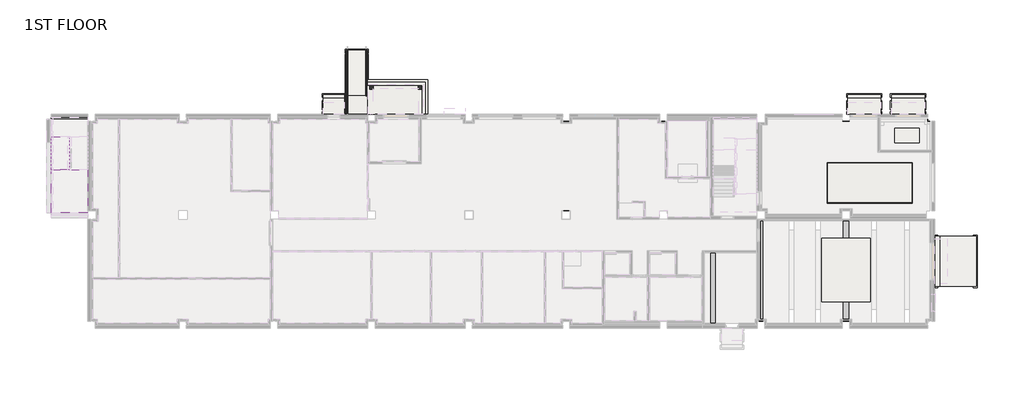
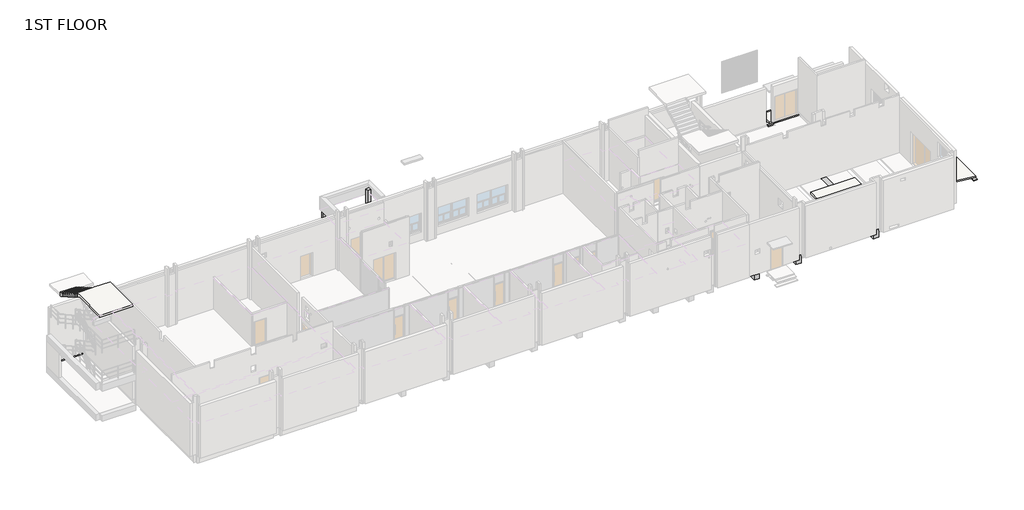
# One storey, part 10 of 15: 37 slabs, 9 beams, 2 columns, 1 stair flight.
# Revit data of these elements (continued)
# Elements 26, 31, 39, 43 (IfcSlab, "H_SF_AR_S18_Lean_T50") (continued)
#   Height Offset From Level = -350 mm
#   built-in parameter 1001954 = 1
#   Phase Created = New Construction
#   Materials on its faces: "Concrete_f'c=14MPa(Cylender)"
# Elements 27, 32, 41 (IfcSlab, "H_SF_AR_S18_Lean_T50")
#   Comments = ""
#   Height Offset From Level = -200 mm
#   built-in parameter 1001954 = 1
#   Phase Created = New Construction
#   Materials on its faces: "Concrete_f'c=14MPa(Cylender)"
# Element 33 (IfcSlab, "H_SF_AR_B08_Stoop_T150")
#   Comments = ""
#   Height Offset From Level = -20 mm
#   built-in parameter 1001954 = 1
#   Phase Created = New Construction
#   Materials on its faces: "Concrete_f'c=28MPa(Cylender)"
# Element 34 (IfcSlab, "H_SF_AR_B08_Stoop_T125")
#   Comments = ""
#   Height Offset From Level = -160 mm
#   built-in parameter 1001954 = 1
#   Phase Created = New Construction
#   Materials on its faces: "Concrete_f'c=28MPa(Cylender)"
# Element 35 (IfcSlab, "H_SF_AR_S18_Lean_T50")
#   Comments = ""
#   Height Offset From Level = -470 mm
#   built-in parameter 1001954 = 1
#   Phase Created = New Construction
#   Materials on its faces: "Concrete_f'c=14MPa(Cylender)"
# Element 36 (IfcSlab, "H_SF_AR_S18_Lean_T50")
#   Comments = ""
#   Height Offset From Level = -320 mm
#   built-in parameter 1001954 = 1
#   Phase Created = New Construction
#   Materials on its faces: "Concrete_f'c=14MPa(Cylender)"
# Element 37 (IfcSlab, "H_SF_AR_S18_Lean_T50")
#   Comments = ""
#   Height Offset From Level = -170 mm
#   built-in parameter 1001954 = 1
#   Phase Created = New Construction
#   Materials on its faces: "Concrete_f'c=14MPa(Cylender)"
# Element 40 (IfcSlab, "H_SF_AR_S18_Lean_T50")
#   Comments = ""
#   Height Offset From Level = -620.333 mm
#   built-in parameter 1001954 = 1
#   Phase Created = New Construction
#   Materials on its faces: "Concrete_f'c=14MPa(Cylender)"
# Element 42 (IfcSlab, "H_SF_AR_S18_Lean_T50")
#   Comments = ""
#   built-in parameter 1001955 = 3.14159 (stored number, unit not read)
#   Height Offset From Level = -350 mm
#   built-in parameter 1001954 = 1
#   Phase Created = New Construction
#   Materials on its faces: "Concrete_f'c=14MPa(Cylender)"
# Elements 44, 45 (IfcSlab, "H_SF_AR_S18_Lean_T50")
#   Comments = ""
#   built-in parameter 1001955 = -1.5708 (stored number, unit not read)
#   Height Offset From Level = -150 mm
#   built-in parameter 1001954 = 1
#   Phase Created = New Construction
#   Materials on its faces: "Concrete_f'c=14MPa(Cylender)"
# Element 46 (IfcSlab, "H_SF_AR_S18_Lean_T50")
#   Comments = ""
#   Height Offset From Level = -450 mm
#   built-in parameter 1001954 = 1
#   Phase Created = New Construction
#   Materials on its faces: "Concrete_f'c=14MPa(Cylender)"
# Element 48 (IfcSlab, "H_SF_AR_S18_Lean_T50")
#   Comments = ""
#   Height Offset From Level = -600 mm
#   built-in parameter 1001954 = 1
#   Phase Created = New Construction
#   Materials on its faces: "Concrete_f'c=14MPa(Cylender)"
# Element 49 (IfcStairFlight, "Concrete")
#   Phase Created = New Construction
#   Materials on its faces: "Concrete_f'c=28MPa(Cylender)"
# Materials
#   "Concrete_f'c=28MPa(Cylender)": class "Concrete", colour RGB 176 176 176, transparency 0, Description = "Reinf. Conc.", Cost = 0, Image = Concrete.Cast-In-Place.Flat.Polished.Grey.jpg
#   "Concrete_f'c=14MPa(Cylender)": class "Concrete", colour RGB 177 177 177, transparency 0, Description = "Reinf. Conc.", Cost = 0
